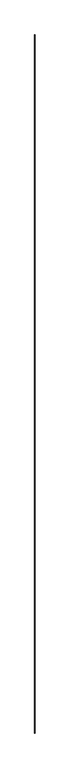
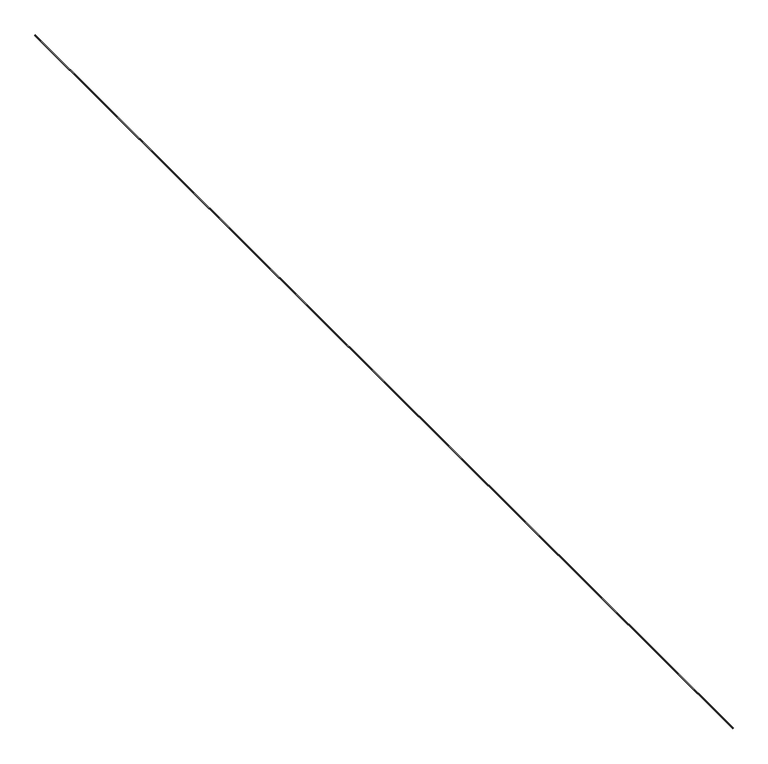
"""IFC4 building model written with IfcOpenShell, lengths in millimetres: proxy geometry, Inner panel:Inner panel:1:Inner panel:1 : Inner panel:Inner panel:300324:2:Inner panel:1:Inner panel:1 : Inner panel:Inner panel:300324:2 : Inner panel:Inner panel:1:Inner panel:1 : Inner panel:Inner panel:300324:300043:58 : Inner panel:Inner panel:1:Inner panel:1 : Inner panel:Inner panel:300324:2:Inner panel:1:Inner panel:1 : Inner panel:Inner panel:300324:2 : Inner panel:Inner panel:1:Inner panel:1 : Inner panel:Inner panel:300324:300043:308120."""

from ifc_helpers import new_model, si_unit, frame, origin, place, context, project, spatial, polyline, outline, extrude, source, transform, mapped, element, save


def generic_models_313c75ba(model_context):
    return source(origin(), model_context, "Body", "SweptSolid", [
        extrude(outline(polyline([(3824.2861619, 558266.1625821), (3825.8722857, 558304.2295522), (3863.9392558, 558302.6434284), (3862.353132, 558264.5764583), (3824.2861619, 558266.1625821)]), holes=[polyline([(3826.7644803, 558268.442635), (3860.0730791, 558267.0547767), (3861.4609374, 558300.3633755), (3828.1523386, 558301.7512338), (3826.7644803, 558268.442635)])]), frame((0.0, -579346.5018006, 0.0), z_axis=(0.0, 1.0, 0.0), x_axis=(0.0, 0.0, 1.0)), (0.0, 0.0, 1.0), 88442.8),
    ])


if __name__ == "__main__":
    model = new_model("IFC4")
    model_context = context("Model", 3, world=origin())
    ifc_project = project(units=[si_unit("LENGTHUNIT", "METRE", prefix="MILLI")], contexts=[model_context])
    site = spatial("IfcSite", under=ifc_project)
    building = spatial("IfcBuilding", under=site)
    placement = place(None, origin())
    generic_models_shape = generic_models_313c75ba(model_context)
    element("IfcBuildingElementProxy", 1, Name="Inner panel:Inner panel:1:Inner panel:1 : Inner panel:Inner panel:300324:2:Inner panel:1:Inner panel:1 : Inner panel:Inner panel:300324:2 : Inner panel:Inner panel:1:Inner panel:1 : Inner panel:Inner panel:300324:300043:58 : Inner panel:Inner panel:1:Inner panel:1 : Inner panel:Inner panel:300324:2:Inner panel:1:Inner panel:1 : Inner panel:Inner panel:300324:2 : Inner panel:Inner panel:1:Inner panel:1 : Inner panel:Inner panel:300324:300043:308120", ObjectType="Inner panel:Inner panel:1:Inner panel:1 : Inner panel:Inner panel:300324:2:Inner panel:1:Inner panel:1 : Inner panel:Inner panel:300324:2 : Inner panel:Inner panel:1:Inner panel:1 : Inner panel:Inner panel:300324:300043:58 : Inner panel:Inner panel:1:Inner panel:1 : Inner panel:Inner panel:300324:2:Inner panel:1:Inner panel:1 : Inner panel:Inner panel:300324:2 : Inner panel:Inner panel:1:Inner panel:1 : Inner panel:Inner panel:300324:300043:308120", at=placement, inside=building, context=model_context, shape_type="MappedRepresentation", body=[
        mapped(generic_models_shape, transform((0.0, 0.0, 0.0), x_axis=(1.0, 0.0, 0.0), y_axis=(0.0, 1.0, 0.0), z_axis=(0.0, 0.0, 1.0))),
    ])
    save(model, "model.ifc")

# Revit data of these elements
# Type "Inner panel:Inner panel:1:Inner panel:1 : Inner panel:Inner panel:300324:2:Inner panel:1:Inner panel:1 : Inner panel:Inner panel:300324:2 : Inner panel:Inner panel:1:Inner panel:1 : Inner panel:Inner panel:300324:300043:58 : Inner panel:Inner panel:1:Inner panel:1 : Inner panel:Inner panel:300324:2:Inner panel:1:Inner panel:1 : Inner panel:Inner panel:300324:2 : Inner panel:Inner panel:1:Inner panel:1 : Inner panel:Inner panel:300324:300043:308120"
#   NameOverride = "Inner panel:Inner panel:1:Inner panel:1 : Inner panel:Inner panel:300324:2:Inner panel:1:Inner panel:1 : Inner panel:Inner panel:300324:2 : Inner panel:Inner panel:1:Inner panel:1 : Inner panel:Inner panel:300324:300043:308120"
#   ObjectTypeOverride = "Inner panel:1:Inner panel:1 : Inner panel:Inner panel:300324:2 : Inner panel:Inner panel:1:Inner panel:1 : Inner panel:Inner panel:300324:300043"
#   Reference = "Inner panel"
#   Tag = "308120"
# Element 1 (IfcBuildingElementProxy, "Inner panel:Inner panel:1:Inner panel:1 : Inner panel:Inner panel:300324:2:Inner panel:1:Inner panel:1 : Inner panel:Inner panel:300324:2 : Inner panel:Inner panel:1:Inner panel:1 : Inner panel:Inner panel:300324:300043:58 : Inner panel:Inner panel:1:Inner panel:1 : Inner panel:Inner panel:300324:2:Inner panel:1:Inner panel:1 : Inner panel:Inner panel:300324:2 : Inner panel:Inner panel:1:Inner panel:1 : Inner panel:Inner panel:300324:300043:308120")
#   Materials on its faces: "1 1/2\" X 1 1/2\" x 1/8\" ALUM. TUBE (6061-T6) - (2) #16 WOOD SCREWS WITH 2.5\" EMBED AT EACH GLULAM - (1) SCREW AT ENDS"
# Materials
#   "1 1/2\" X 1 1/2\" x 1/8\" ALUM. TUBE (6061-T6) - (2) #16 WOOD SCREWS WITH 2.5\" EMBED AT EACH GLULAM - (1) SCREW AT ENDS": class "Unassigned", colour RGB 202 201 200, transparency 0, Cost = 0
